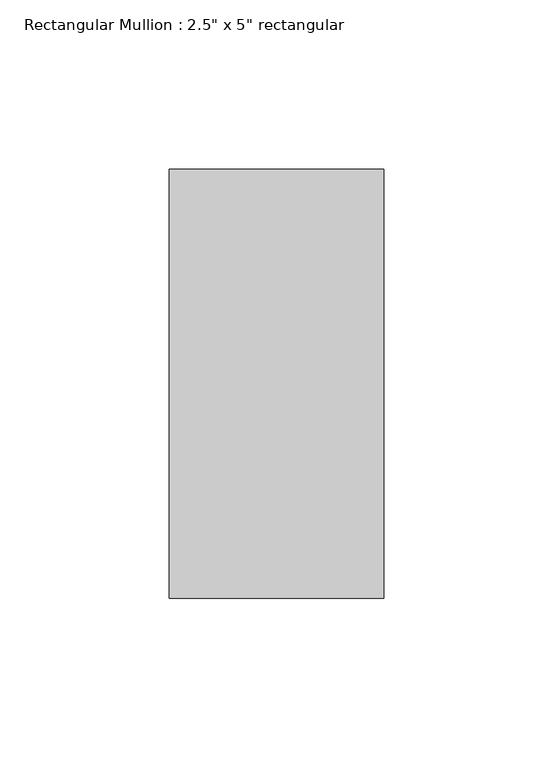
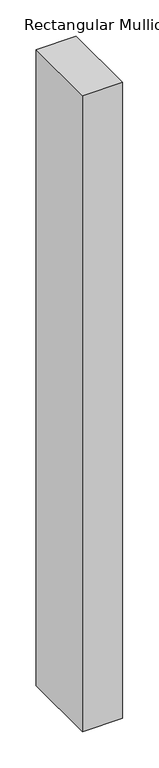
"""IFC4 building model written with IfcOpenShell, lengths in millimetres: member geometry."""

from ifc_helpers import new_model, si_unit, frame, origin, place, context, project, spatial, polyline, outline, extrude, source, transform, mapped, element, save


def member_c4de40ee(model_context):
    return source(origin(), model_context, "Body", "SweptSolid", [
        extrude(outline(polyline([(0.0, 63.5), (0.0, -63.5), (-63.5, -63.5), (-63.5, 63.5), (0.0, 63.5)])), frame((0.0, 0.0, -1066.8), z_axis=(0.0, 0.0, 1.0), x_axis=(1.0, 0.0, 0.0)), (0.0, 0.0, 1.0), 1066.8),
    ])


if __name__ == "__main__":
    model = new_model("IFC4")
    model_context = context("Model", 3, world=origin())
    ifc_project = project(units=[si_unit("LENGTHUNIT", "METRE", prefix="MILLI")], contexts=[model_context])
    site = spatial("IfcSite", under=ifc_project)
    building = spatial("IfcBuilding", under=site)
    placement = place(None, origin())
    member_shape = member_c4de40ee(model_context)
    element("IfcMember", 1, ObjectType="Rectangular Mullion : 2.5\" x 5\" rectangular", at=placement, inside=building, context=model_context, shape_type="MappedRepresentation", body=[
        mapped(member_shape, transform((0.0, 0.0, 0.0), x_axis=(1.0, 0.0, 0.0), y_axis=(0.0, 1.0, 0.0), z_axis=(0.0, 0.0, 1.0))),
    ])
    save(model, "model.ifc")

# Revit data of these elements
# Type "Rectangular Mullion : 2.5\" x 5\" rectangular"
#   built-in parameter 1007304 = 0.416667 (stored number, unit not read)
#   built-in parameter 1007301 = 0.104167 (stored number, unit not read)
#   built-in parameter 1007300 = 0.104167 (stored number, unit not read)
# Element 1 (IfcMember, "Rectangular Mullion : 2.5\" x 5\" rectangular")
#   Materials on its faces: "Metal - Aluminum"
# Materials
#   "Metal - Aluminum": class "Metal", colour RGB 140 140 140, transparency 0
